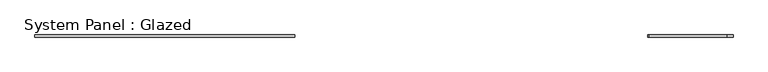
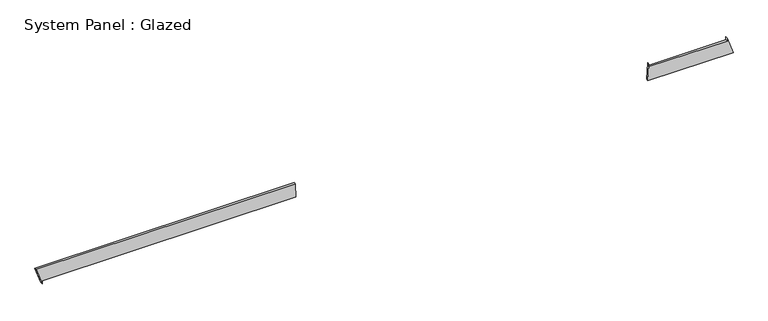
"""IFC4 building model written with IfcOpenShell, lengths in millimetres: plate geometry, System Panel : Glazed."""

from ifc_helpers import new_model, si_unit, frame, origin, place, context, project, spatial, polyline, outline, extrude, source, transform, mapped, element, save


def system_panel_glazed_f2b34a5e(model_context):
    return source(origin(), model_context, "Body", "SweptSolid", [
        extrude(outline(polyline([(35.3553391, 3043.6334639), (35.3553391, 4027.4732247), (235.6210783, 3958.4712631), (200.2657393, 3958.4719436), (200.2483347, 3054.1964159), (235.6036737, 3054.1957354), (35.3553391, 3043.6334639)])), frame((0.0, -49.5, 0.0), z_axis=(0.0, 1.0, 0.0), x_axis=(0.0, 0.0, 1.0)), (0.0, 0.0, 1.0), 25.0),
        extrude(outline(polyline([(0.0, -3958.100606), (35.3553391, -3958.100606), (35.3553391, -1029.4125478), (200.1696818, -1032.3090079), (200.1120339, -4027.4732247), (0.0, -3958.100606)])), frame((0.0, -49.5, 0.0), z_axis=(0.0, 1.0, 0.0), x_axis=(0.0, 0.0, 1.0)), (0.0, 0.0, 1.0), 25.0),
    ])


if __name__ == "__main__":
    model = new_model("IFC4")
    model_context = context("Model", 3, world=origin())
    ifc_project = project(units=[si_unit("LENGTHUNIT", "METRE", prefix="MILLI")], contexts=[model_context])
    site = spatial("IfcSite", under=ifc_project)
    building = spatial("IfcBuilding", under=site)
    placement = place(None, origin())
    system_panel_glazed_shape = system_panel_glazed_f2b34a5e(model_context)
    element("IfcPlate", 1, ObjectType="System Panel : Glazed", at=placement, inside=building, context=model_context, shape_type="MappedRepresentation", body=[
        mapped(system_panel_glazed_shape, transform((0.0, 0.0, 0.0), x_axis=(1.0, 0.0, 0.0), y_axis=(0.0, 1.0, 0.0), z_axis=(0.0, 0.0, 1.0))),
    ])
    save(model, "model.ifc")

# Revit data of these elements
# Element 1 (IfcPlate, "System Panel : Glazed")
#   Materials on its faces: "Glass"
# Materials
#   "Glass": class "Glass", colour RGB 218 227 224, transparency 0.85, Description = "Soda Lime Glass", Cost = 0
